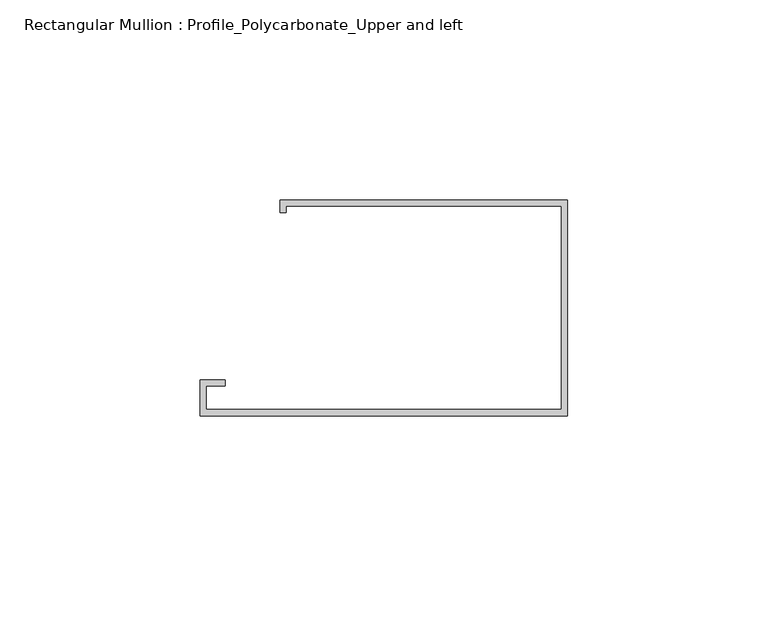
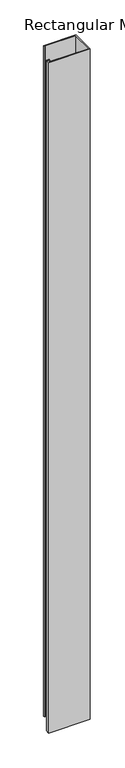
"""IFC4 building model written with IfcOpenShell, lengths in millimetres: member geometry, Rectangular Mullion : Profile_Polycarbonate_Upper and left."""

from ifc_helpers import new_model, si_unit, frame, origin, place, context, project, spatial, polyline, outline, extrude, source, transform, mapped, element, save


def rectangular_mullion_profile_polycarbonate_upper_and_left_2c8d73ac(model_context):
    return source(origin(), model_context, "Body", "SweptSolid", [
        extrude(outline(polyline([(0.0, -28.984575), (-91.9988, -28.984575), (-91.9988, -19.992975), (-85.6488, -19.992975), (-85.6488, -21.580475), (-90.4113, -21.580475), (-90.4113, -27.397075), (-1.5875, -27.397075), (-1.5875, 23.428325), (-70.3961, 23.428325), (-70.3961, 21.840825), (-71.9836, 21.840825), (-71.9836, 25.015825), (0.0, 25.015825), (0.0, -28.984575)])), frame((0.0, 0.0, -1576.0090389), z_axis=(0.0, 0.0, 1.0), x_axis=(1.0, 0.0, 0.0)), (0.0, 0.0, 1.0), 1576.0090389),
    ])


if __name__ == "__main__":
    model = new_model("IFC4")
    model_context = context("Model", 3, world=origin())
    ifc_project = project(units=[si_unit("LENGTHUNIT", "METRE", prefix="MILLI")], contexts=[model_context])
    site = spatial("IfcSite", under=ifc_project)
    building = spatial("IfcBuilding", under=site)
    placement = place(None, origin())
    rectangular_mullion_profile_polycarbonate_upper_and_left_shape = rectangular_mullion_profile_polycarbonate_upper_and_left_2c8d73ac(model_context)
    element("IfcMember", 1, ObjectType="Rectangular Mullion : Profile_Polycarbonate_Upper and left", at=placement, inside=building, context=model_context, shape_type="MappedRepresentation", body=[
        mapped(rectangular_mullion_profile_polycarbonate_upper_and_left_shape, transform((0.0, 0.0, 0.0), x_axis=(1.0, 0.0, 0.0), y_axis=(0.0, 1.0, 0.0), z_axis=(0.0, 0.0, 1.0))),
    ])
    save(model, "model.ifc")

# Revit data of these elements
# Type "Rectangular Mullion : Profile_Polycarbonate_Upper and left"
#   built-in parameter 1007322 = 0.177167 (stored number, unit not read)
#   built-in parameter 1007321 = 0.00520833 (stored number, unit not read)
#   built-in parameter 1007320 = 0 (stored number, unit not read)
